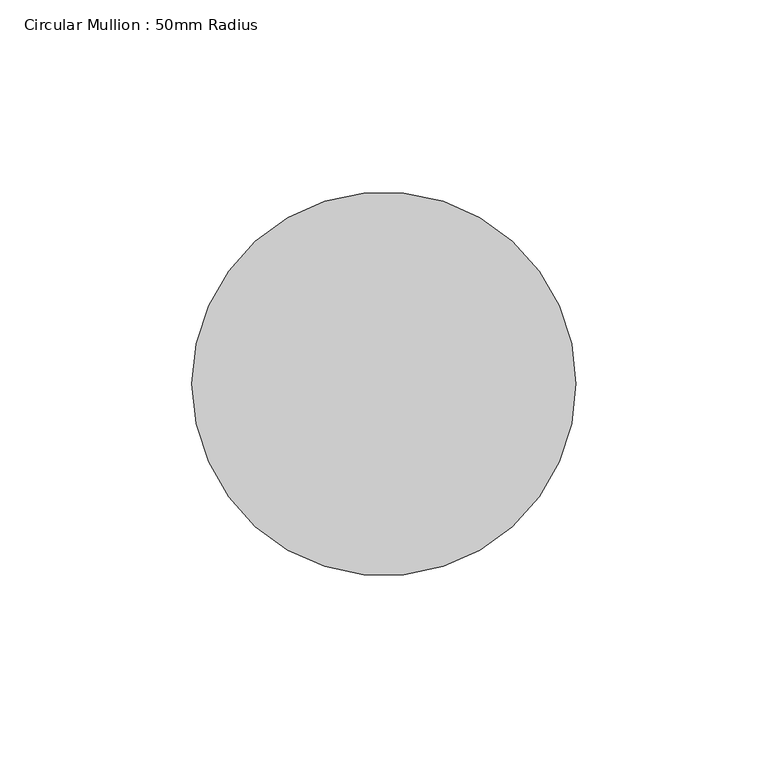
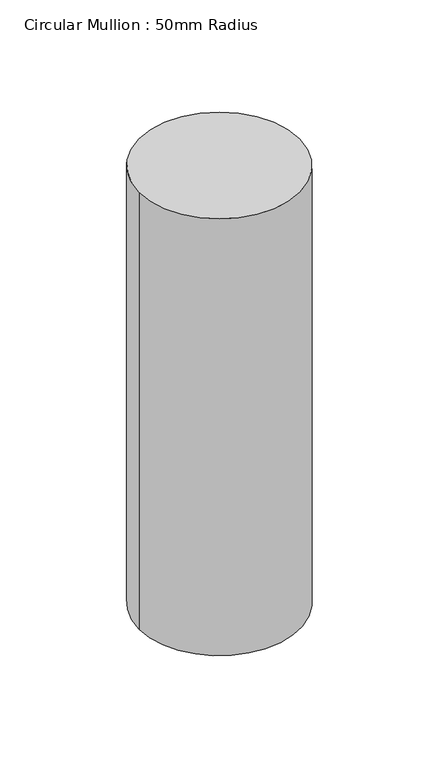
"""IFC4 building model written with IfcOpenShell, lengths in millimetres: member geometry, Circular Mullion : 50mm Radius."""

from ifc_helpers import new_model, si_unit, point, frame, origin, origin_2d, place, context, project, spatial, circle_curve, trimmed, segment, composite_curve, outline, extrude, source, transform, mapped, element, save


def circular_mullion_50mm_radius_c332403b(model_context):
    return source(origin(), model_context, "Body", "SweptSolid", [
        extrude(outline(composite_curve([segment(trimmed(circle_curve(origin_2d(), 50.0), [point((50.0, 0.0))], [point((-50.0, 0.0))], False, "CARTESIAN"), True, "CONTINUOUS"), segment(trimmed(circle_curve(origin_2d(), 50.0), [point((-50.0, 0.0))], [point((50.0, 0.0))], False, "CARTESIAN"), True, "CONTINUOUS")], self_intersect=False)), frame((0.0, 0.0, -287.4913253), z_axis=(0.0, 0.0, 1.0), x_axis=(1.0, 0.0, 0.0)), (0.0, 0.0, 1.0), 287.4913253),
    ])


if __name__ == "__main__":
    model = new_model("IFC4")
    model_context = context("Model", 3, world=origin())
    ifc_project = project(units=[si_unit("LENGTHUNIT", "METRE", prefix="MILLI")], contexts=[model_context])
    site = spatial("IfcSite", under=ifc_project)
    building = spatial("IfcBuilding", under=site)
    placement = place(None, origin())
    circular_mullion_50mm_radius_shape = circular_mullion_50mm_radius_c332403b(model_context)
    element("IfcMember", 1, ObjectType="Circular Mullion : 50mm Radius", at=placement, inside=building, context=model_context, shape_type="MappedRepresentation", body=[
        mapped(circular_mullion_50mm_radius_shape, transform((0.0, 0.0, 0.0), x_axis=(1.0, 0.0, 0.0), y_axis=(0.0, 1.0, 0.0), z_axis=(0.0, 0.0, 1.0))),
    ])
    save(model, "model.ifc")

# Revit data of these elements
# Type "Circular Mullion : 50mm Radius"
#   built-in parameter 1007350 = 0.164042 (stored number, unit not read)
# Element 1 (IfcMember, "Circular Mullion : 50mm Radius")
#   Materials on its faces: "Aluminium"
# Materials
#   "Aluminium": class "Metal", colour RGB 247 247 247, transparency 0, Description = "Aluminium 6061", Cost = 0
